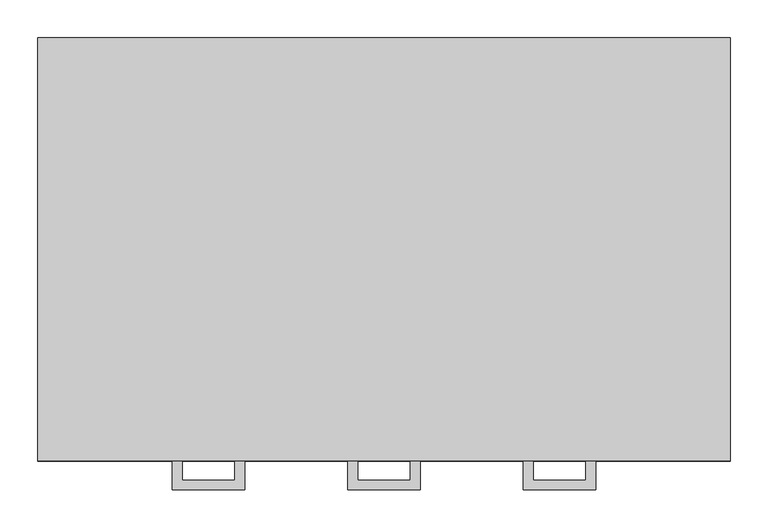
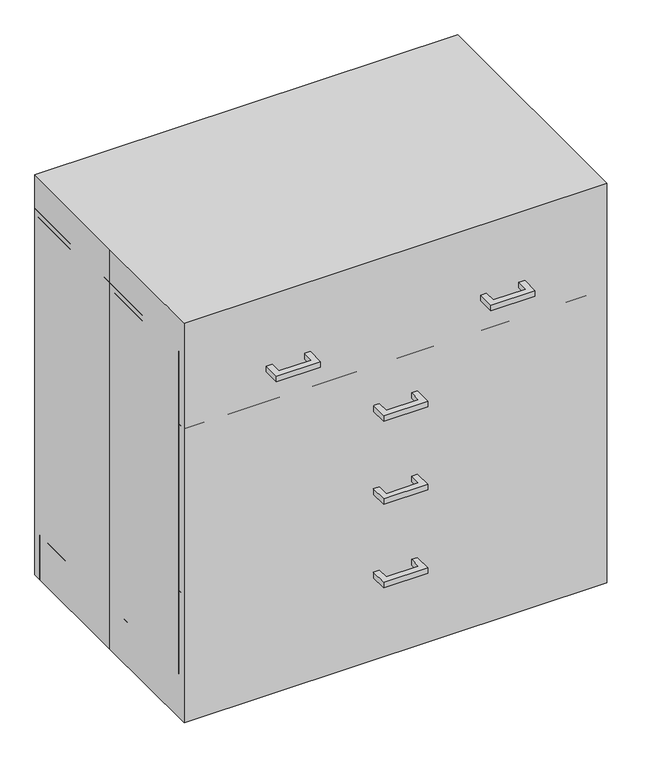
"""IFC4 building model written with IfcOpenShell, lengths in millimetres: proxy geometry, C04H0 - Cabinet, U-C-B, 2 Half DR, 3 DR, 36x36x22 : C04H0 - Cabinet, U-C-B, 2 Half DR, 3 DR, 36x36x22."""

import ifcopenshell
import ifcopenshell.guid

model = None  # the IFC model being written
_history = None  # IfcOwnerHistory: only IFC2X3 demands one
_inside = {}  # id of a spatial element -> (the spatial element, [elements in it])
_under = {}  # id of a project, library or spatial element -> (it, [spatial elements below it])
_declared = {}  # id of a project -> (the project, [libraries it declares])
_typed = {}  # id of a type object -> (the type object, [elements of that type])
_made_of = {}  # id of a material, layer set ... -> (it, [elements and type objects made of it])


def new_model(schema):
    """Start an empty IFC model of exactly this schema.

    Asked for "IFC4X3", IfcOpenShell would pick the latest addendum, in which some entities
    have other attributes; the version numbers below select the first issue.
    IFC2X3 requires an IfcOwnerHistory on every rooted entity: one is made here for all.
    """
    global model, _history
    if schema == "IFC4X3":
        model = ifcopenshell.file(schema_version=(4, 3, 0, 0))
    else:
        model = ifcopenshell.file(schema=schema)
    _inside.clear()
    _under.clear()
    _declared.clear()
    _typed.clear()
    _made_of.clear()
    _history = None
    if model.schema == "IFC2X3":
        org = make("IfcOrganization", Name="unknown")
        user = make(
            "IfcPersonAndOrganization",
            ThePerson=make("IfcPerson", FamilyName="unknown"),
            TheOrganization=org,
        )
        app = make(
            "IfcApplication",
            ApplicationDeveloper=org,
            Version="unknown",
            ApplicationFullName="unknown",
            ApplicationIdentifier="unknown",
        )
        _history = make(
            "IfcOwnerHistory",
            OwningUser=user,
            OwningApplication=app,
            ChangeAction="ADDED",
            CreationDate=0,
        )
    return model


def make(cls, **values):
    """One entity of the class cls with the attributes given. An attribute that is None is left unset."""
    return model.create_entity(
        cls, **{name: value for name, value in values.items() if value is not None}
    )


def rooted(cls, **values):
    """An entity with a GlobalId (a new one), such as an element, a storey or a relation."""
    return make(cls, GlobalId=ifcopenshell.guid.new(), OwnerHistory=_history, **values)


def si_unit(unit_type, name, prefix=None):
    """IfcSIUnit, for example si_unit("LENGTHUNIT", "METRE", prefix="MILLI")."""
    return make("IfcSIUnit", UnitType=unit_type, Prefix=prefix, Name=name)


def assignment(units):
    """IfcUnitAssignment: the units of a project."""
    return None if units is None else make("IfcUnitAssignment", Units=units)


def point(xyz):
    """IfcCartesianPoint."""
    return None if xyz is None else make("IfcCartesianPoint", Coordinates=xyz)


def direction(xyz):
    """IfcDirection."""
    return None if xyz is None else make("IfcDirection", DirectionRatios=xyz)


def frame(location, z_axis=None, x_axis=None):
    """IfcAxis2Placement3D, a coordinate frame: its origin and axes. An axis left out is left unset."""
    return make(
        "IfcAxis2Placement3D",
        Location=point(location),
        Axis=direction(z_axis),
        RefDirection=direction(x_axis),
    )


def origin():
    """The frame at (0, 0, 0) with its axes left unset."""
    return frame((0.0, 0.0, 0.0))


def origin_with_axes():
    """The frame at (0, 0, 0) with the z axis (0, 0, 1) and the x axis (1, 0, 0) written out."""
    return frame((0.0, 0.0, 0.0), z_axis=(0.0, 0.0, 1.0), x_axis=(1.0, 0.0, 0.0))


def place(relative_to, where):
    """IfcLocalPlacement: puts the frame where relative to a parent placement (None: the world)."""
    return make(
        "IfcLocalPlacement", PlacementRelTo=relative_to, RelativePlacement=where
    )


def context(
    kind, dimensions, precision=None, world=None, true_north=None, identifier=None
):
    """IfcGeometricRepresentationContext, for example the 3D "Model" context."""
    return make(
        "IfcGeometricRepresentationContext",
        ContextIdentifier=identifier,
        ContextType=kind,
        CoordinateSpaceDimension=dimensions,
        Precision=precision,
        WorldCoordinateSystem=world,
        TrueNorth=true_north,
    )


def project(units=None, contexts=None):
    """IfcProject with its units and contexts."""
    return rooted(
        "IfcProject",
        Name="project",
        RepresentationContexts=contexts,
        UnitsInContext=assignment(units),
    )


def spatial(cls, under=None, at=None, **own):
    """A site, building, storey or space (cls), placed at a placement, below another one or the project."""
    s = rooted(cls, ObjectPlacement=at, **own)
    if under is not None:
        _under.setdefault(under.id(), (under, []))[1].append(s)
    return s


def polyline(points):
    """IfcPolyline through the points."""
    return make("IfcPolyline", Points=[point(p) for p in points])


def outline(outer, holes=None, kind="AREA"):
    """IfcArbitraryClosedProfileDef: a profile drawn as a closed curve; with holes, ...WithVoids."""
    if holes is None:
        return make("IfcArbitraryClosedProfileDef", ProfileType=kind, OuterCurve=outer)
    return make(
        "IfcArbitraryProfileDefWithVoids",
        ProfileType=kind,
        OuterCurve=outer,
        InnerCurves=holes,
    )


def extrude(swept, where, along, depth):
    """IfcExtrudedAreaSolid: the profile swept, set in the frame where, extruded along a direction by depth."""
    return make(
        "IfcExtrudedAreaSolid",
        SweptArea=swept,
        Position=where,
        ExtrudedDirection=direction(along),
        Depth=depth,
    )


def shape(context_of_items, identifier, shape_type, items):
    """IfcShapeRepresentation: the items that make up one representation, for example the "Body"."""
    return make(
        "IfcShapeRepresentation",
        ContextOfItems=context_of_items,
        RepresentationIdentifier=identifier,
        RepresentationType=shape_type,
        Items=items,
    )


def source(mapping_origin, context_of_items, identifier, shape_type, items):
    """IfcRepresentationMap: a shape defined once, which mapped items show again and again."""
    return make(
        "IfcRepresentationMap",
        MappingOrigin=mapping_origin,
        MappedRepresentation=shape(context_of_items, identifier, shape_type, items),
    )


def transform(
    local_origin,
    x_axis=None,
    y_axis=None,
    z_axis=None,
    scale=None,
    scale2=None,
    scale3=None,
    uniform=True,
):
    """IfcCartesianTransformationOperator3D, or its non-uniform kind. x_axis, y_axis, z_axis: its Axis1, 2, 3."""
    if uniform:
        return make(
            "IfcCartesianTransformationOperator3D",
            Axis1=direction(x_axis),
            Axis2=direction(y_axis),
            LocalOrigin=point(local_origin),
            Scale=scale,
            Axis3=direction(z_axis),
        )
    return make(
        "IfcCartesianTransformationOperator3DnonUniform",
        Axis1=direction(x_axis),
        Axis2=direction(y_axis),
        LocalOrigin=point(local_origin),
        Scale=scale,
        Axis3=direction(z_axis),
        Scale2=scale2,
        Scale3=scale3,
    )


def mapped(mapping_source, mapping_target):
    """IfcMappedItem: shows the shape of a source again, moved by a transform."""
    return make(
        "IfcMappedItem", MappingSource=mapping_source, MappingTarget=mapping_target
    )


def made_of(thing, what):
    """Note that an element or type object is made of a material, layer set ...; save() writes the relation."""
    if what is not None:
        _made_of.setdefault(what.id(), (what, []))[1].append(thing)
    return thing


def element(
    cls,
    number,
    at=None,
    inside=None,
    cuts=None,
    type_object=None,
    material=None,
    context=None,
    identifier="Body",
    shape_type=None,
    held_by="IfcProductDefinitionShape",
    body=None,
    shapes=None,
    **own,
):
    """One element of the class cls, such as IfcWall. Its Tag is "e" and its number.

    at: its placement. inside: the storey or other place that contains it. cuts: it is an
    opening in that element (IfcRelVoidsElement). A single representation is given by context,
    identifier, shape_type and body (its items); several are given by shapes. held_by: the class
    of the entity that holds the representations. save() writes the other relations.
    """
    e = rooted(cls, Tag="e%d" % number, ObjectPlacement=at, **own)
    if body is not None:
        shapes = [shape(context, identifier, shape_type, body)]
    if shapes is not None:
        e.Representation = make(held_by, Representations=shapes)
    if inside is not None:
        _inside.setdefault(inside.id(), (inside, []))[1].append(e)
    if cuts is not None:
        rooted(
            "IfcRelVoidsElement", RelatingBuildingElement=cuts, RelatedOpeningElement=e
        )
    if type_object is not None:
        _typed.setdefault(type_object.id(), (type_object, []))[1].append(e)
    return made_of(e, material)


def aggregate(whole, parts):
    """IfcRelAggregates: a whole, such as a stair, and the parts it consists of."""
    return rooted("IfcRelAggregates", RelatingObject=whole, RelatedObjects=parts)


def save(model, path):
    """Write the relations noted so far, then the file.

    IfcRelAggregates (storeys below a building ...), IfcRelContainedInSpatialStructure (elements
    in a storey), IfcRelDefinesByType, IfcRelAssociatesMaterial and IfcRelDeclares: one each for
    every whole, place, type object, material and project.
    """
    for whole, parts in _under.values():
        aggregate(whole, parts)
    for where, things in _inside.values():
        rooted(
            "IfcRelContainedInSpatialStructure",
            RelatedElements=things,
            RelatingStructure=where,
        )
    for kind, things in _typed.values():
        rooted("IfcRelDefinesByType", RelatedObjects=things, RelatingType=kind)
    for what, things in _made_of.values():
        rooted("IfcRelAssociatesMaterial", RelatedObjects=things, RelatingMaterial=what)
    for by, libraries in _declared.values():
        rooted("IfcRelDeclares", RelatingContext=by, RelatedDefinitions=libraries)
    model.write(path)


def specialty_equipment_32dd883c(model_context):
    return source(origin(), model_context, "Body", "SweptSolid", [
        extrude(outline(polyline([(-47.625, -317.5), (-47.625, -279.4), (-34.9409299, -279.4), (-34.9409299, -304.8159299), (34.9409299, -304.8159299), (34.9409299, -279.4), (47.625, -279.4), (47.625, -317.5), (-47.625, -317.5)])), frame((0.0, 0.0, 188.8962383), z_axis=(0.0, 0.0, 1.0), x_axis=(1.0, 0.0, 0.0)), (0.0, 0.0, 1.0), 12.7),
        extrude(outline(polyline([(-47.625, -317.5), (-47.625, -279.4), (-34.9409299, -279.4), (-34.9409299, -304.8159299), (34.9409299, -304.8159299), (34.9409299, -279.4), (47.625, -279.4), (47.625, -317.5), (-47.625, -317.5)])), frame((0.0, 0.0, 379.3962383), z_axis=(0.0, 0.0, 1.0), x_axis=(1.0, 0.0, 0.0)), (0.0, 0.0, 1.0), 12.7),
        extrude(outline(polyline([(-47.625, -317.5), (-47.625, -279.4), (-34.9409299, -279.4), (-34.9409299, -304.8159299), (34.9409299, -304.8159299), (34.9409299, -279.4), (47.625, -279.4), (47.625, -317.5), (-47.625, -317.5)])), frame((0.0, 0.0, 569.8962383), z_axis=(0.0, 0.0, 1.0), x_axis=(1.0, 0.0, 0.0)), (0.0, 0.0, 1.0), 12.7),
        extrude(outline(polyline([(-279.3840701, -317.5), (-279.3840701, -279.4), (-266.7, -279.4), (-266.7, -304.8159299), (-196.8181401, -304.8159299), (-196.8181401, -279.4), (-184.1340701, -279.4), (-184.1340701, -317.5), (-279.3840701, -317.5)])), frame((0.0, 0.0, 741.3462383), z_axis=(0.0, 0.0, 1.0), x_axis=(1.0, 0.0, 0.0)), (0.0, 0.0, 1.0), 12.7),
        extrude(outline(polyline([(279.3840701, -317.5), (184.1340701, -317.5), (184.1340701, -279.4), (196.8181401, -279.4), (196.8181401, -304.8159299), (266.7, -304.8159299), (266.7, -279.4), (279.3840701, -279.4), (279.3840701, -317.5)])), frame((0.0, 0.0, 741.3462383), z_axis=(0.0, 0.0, 1.0), x_axis=(1.0, 0.0, 0.0)), (0.0, 0.0, 1.0), 12.7),
        extrude(outline(polyline([(-457.2, 279.4), (457.2, 279.4), (457.2, -279.4), (-457.2, -279.4), (-457.2, 0.0), (-457.2, 279.4)])), origin_with_axes(), (0.0, 0.0, 1.0), 914.4),
        extrude(outline(polyline([(457.2, -279.4), (-457.2, -279.4), (-457.2, -260.35), (457.2, -260.35), (457.2, -279.4)])), frame((0.0, 0.0, 101.5674767), z_axis=(0.0, 0.0, 1.0), x_axis=(1.0, 0.0, 0.0)), (0.0, 0.0, 1.0), 190.5),
        extrude(outline(polyline([(457.2, -279.4), (-457.2, -279.4), (-457.2, -260.35), (457.2, -260.35), (457.2, -279.4)])), frame((0.0, 0.0, 292.0674767), z_axis=(0.0, 0.0, 1.0), x_axis=(1.0, 0.0, 0.0)), (0.0, 0.0, 1.0), 190.5),
        extrude(outline(polyline([(457.2, -279.4), (-457.2, -279.4), (-457.2, -260.35), (457.2, -260.35), (457.2, -279.4)])), frame((0.0, 0.0, 482.5674767), z_axis=(0.0, 0.0, 1.0), x_axis=(1.0, 0.0, 0.0)), (0.0, 0.0, 1.0), 190.5),
        extrude(outline(polyline([(457.2, -279.4), (0.0, -279.4), (0.0, -260.35), (457.2, -260.35), (457.2, -279.4)])), frame((0.0, 0.0, 673.0674767), z_axis=(0.0, 0.0, 1.0), x_axis=(1.0, 0.0, 0.0)), (0.0, 0.0, 1.0), 152.4),
        extrude(outline(polyline([(0.0, -279.4), (-457.2, -279.4), (-457.2, -260.35), (0.0, -260.35), (0.0, -279.4)])), frame((0.0, 0.0, 673.0674767), z_axis=(0.0, 0.0, 1.0), x_axis=(1.0, 0.0, 0.0)), (0.0, 0.0, 1.0), 152.4),
        extrude(outline(polyline([(-457.2, -260.35), (-457.2, 279.4), (-438.15, 279.4), (-438.15, -260.35), (-457.2, -260.35)])), frame((0.0, 0.0, 101.6), z_axis=(0.0, 0.0, 1.0), x_axis=(1.0, 0.0, 0.0)), (0.0, 0.0, 1.0), 723.8674767),
        extrude(outline(polyline([(438.15, -260.35), (438.15, 279.4), (457.2, 279.4), (457.2, -260.35), (438.15, -260.35)])), frame((0.0, 0.0, 101.6), z_axis=(0.0, 0.0, 1.0), x_axis=(1.0, 0.0, 0.0)), (0.0, 0.0, 1.0), 723.8674767),
        extrude(outline(polyline([(457.2, 279.4), (457.2, -260.35), (-457.2, -260.35), (-457.2, 279.4), (457.2, 279.4)])), frame((0.0, 0.0, 825.4674767), z_axis=(0.0, 0.0, 1.0), x_axis=(1.0, 0.0, 0.0)), (0.0, 0.0, 1.0), 12.7325233),
        extrude(outline(polyline([(457.2, -203.2), (-457.2, -203.2), (-457.2, -184.15), (457.2, -184.15), (457.2, -203.2)])), origin_with_axes(), (0.0, 0.0, 1.0), 101.6),
        extrude(outline(polyline([(-457.2, -184.15), (-457.2, 279.4), (-438.15, 279.4), (-438.15, -184.15), (-457.2, -184.15)])), origin_with_axes(), (0.0, 0.0, 1.0), 101.6),
        extrude(outline(polyline([(438.15, -184.15), (438.15, 279.4), (457.2, 279.4), (457.2, -184.15), (438.15, -184.15)])), origin_with_axes(), (0.0, 0.0, 1.0), 101.6),
        extrude(outline(polyline([(457.2, 260.35), (-457.2, 260.35), (-457.2, 279.4), (457.2, 279.4), (457.2, 260.35)])), origin_with_axes(), (0.0, 0.0, 1.0), 101.6),
        extrude(outline(polyline([(438.15, 260.35), (438.15, -260.35), (-438.15, -260.35), (-438.15, 260.35), (438.15, 260.35)])), frame((0.0, 0.0, 101.6), z_axis=(0.0, 0.0, 1.0), x_axis=(1.0, 0.0, 0.0)), (0.0, 0.0, 1.0), 19.1166954),
        extrude(outline(polyline([(438.15, 260.35), (-438.15, 260.35), (-438.15, 279.4), (438.15, 279.4), (438.15, 260.35)])), frame((0.0, 0.0, 101.6), z_axis=(0.0, 0.0, 1.0), x_axis=(1.0, 0.0, 0.0)), (0.0, 0.0, 1.0), 704.8174767),
    ])


if __name__ == "__main__":
    model = new_model("IFC4")
    model_context = context("Model", 3, world=origin())
    ifc_project = project(units=[si_unit("LENGTHUNIT", "METRE", prefix="MILLI")], contexts=[model_context])
    site = spatial("IfcSite", under=ifc_project)
    building = spatial("IfcBuilding", under=site)
    placement = place(None, origin())
    specialty_equipment_shape = specialty_equipment_32dd883c(model_context)
    element("IfcBuildingElementProxy", 1, Name="C04H0 - Cabinet, U-C-B, 2 Half DR, 3 DR, 36x36x22 : C04H0 - Cabinet, U-C-B, 2 Half DR, 3 DR, 36x36x22", ObjectType="C04H0 - Cabinet, U-C-B, 2 Half DR, 3 DR, 36x36x22 : C04H0 - Cabinet, U-C-B, 2 Half DR, 3 DR, 36x36x22", at=placement, inside=building, context=model_context, shape_type="MappedRepresentation", body=[
        mapped(specialty_equipment_shape, transform((0.0, 0.0, 0.0), x_axis=(1.0, 0.0, 0.0), y_axis=(0.0, 1.0, 0.0), z_axis=(0.0, 0.0, 1.0))),
    ])
    save(model, "model.ifc")

# Revit data of these elements
# Project information
#   Sheets - Total = "6"
#   Project Issue Date = "Issue Date"
#   Project Status = "Project Status"
#   Client Name = "Owner"
#   Project Address = "Enter address here"
#   Project Name = "Project Name"
#   Project Number = "Project Number"
#   Publication Date = "1-Feb-16"
# Type "C04H0 - Cabinet, U-C-B, 2 Half DR, 3 DR, 36x36x22 : C04H0 - Cabinet, U-C-B, 2 Half DR, 3 DR, 36x36x22"
#   Watts2 = "0"
#   Watts1 = "0"
#   Unit_Issue = "EA"
#   UTIL_6_Misc = "-"
#   UTIL_5_NonMedGas = "-"
#   UTIL_4_MiscGas = "-"
#   UTIL_3_MedGas = "-"
#   UTIL_2_Elec = "-"
#   UTIL_1_WaterDrain = "-"
#   Nomenclature = "Cabinet, U/C/B, 2 Half Drawer, 3 Drawer, 36x36x22"
#   NSN = "6530"
#   Location [instance default] = ""
#   JSN = "C04H0"
#   Fund_Source_VA = "-"
#   Fund_Source_Navy = "-"
#   Fund_Source_Army = "-"
#   Fund_Source_AF = "-"
#   ELEC_Volts2 = "0"
#   ELEC_Volts1 = "0"
#   ELEC_Phase2 = "0"
#   ELEC_Phase1 = "0"
#   ELEC_HertzSwitch = "0"
#   ELEC_HertzDependent = "0"
#   ELEC_Hertz = "0"
#   ELEC_Amps2 = "0"
#   ELEC_Amps1 = "0"
#   DetailDescription = "Standing height under counter base cabinet with two half width drawers side-by-side above three full width drawers. Also referred to as a drawer cabinet. For general purpose use throughout the facility."
#   CAT_VA = "A"
#   CAT_Navy = "A"
#   CAT_IHS = "-"
#   CAT_Army = "A"
#   CAT_AF = "A"
#   BTUperhour = "0"
#   Weight_IP = 155
#   DIM_Width_IP = 3' - 0"
#   DIM_Height_IP = 3' - 0"
#   DIM_Depth_IP = 1' - 10"
#   Top Panel Material = none
#   Toe Panel Material = none
#   Side Panel Material = none
#   Shelf Panel Material = none
#   Drawer Front Material = none
#   Door Panel Material = none
#   Back Panel Material = none
#   Assembly Code = ""
# Element 1 (IfcBuildingElementProxy, "C04H0 - Cabinet, U-C-B, 2 Half DR, 3 DR, 36x36x22 : C04H0 - Cabinet, U-C-B, 2 Half DR, 3 DR, 36x36x22")
#   Materials on its faces: "Default metal", "EquipSpace"
# Materials
#   "Default metal": class "Unassigned", colour RGB 204 204 204, transparency 0
#   "EquipSpace": class "Unassigned", colour RGB 221 217 195, transparency 0.5
